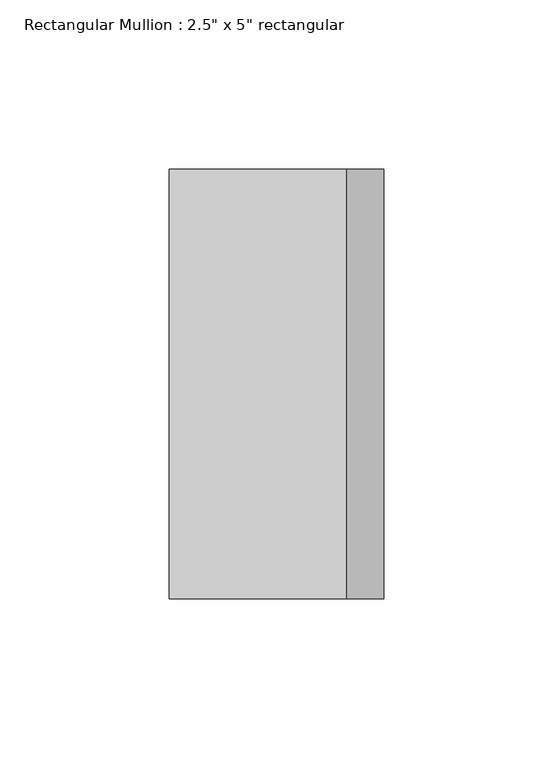
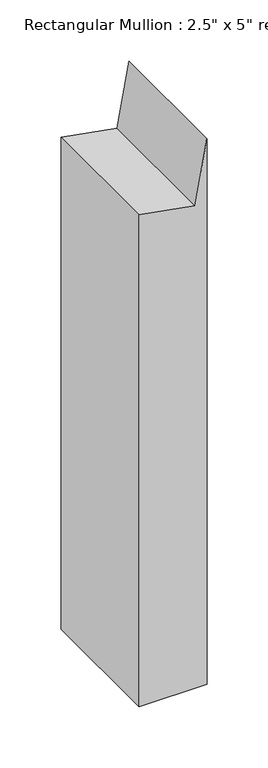
"""IFC4 building model written with IfcOpenShell, lengths in millimetres: member geometry."""

import ifcopenshell
import ifcopenshell.guid

model = None  # the IFC model being written
_history = None  # IfcOwnerHistory: only IFC2X3 demands one
_inside = {}  # id of a spatial element -> (the spatial element, [elements in it])
_under = {}  # id of a project, library or spatial element -> (it, [spatial elements below it])
_declared = {}  # id of a project -> (the project, [libraries it declares])
_typed = {}  # id of a type object -> (the type object, [elements of that type])
_made_of = {}  # id of a material, layer set ... -> (it, [elements and type objects made of it])


def new_model(schema):
    """Start an empty IFC model of exactly this schema.

    Asked for "IFC4X3", IfcOpenShell would pick the latest addendum, in which some entities
    have other attributes; the version numbers below select the first issue.
    IFC2X3 requires an IfcOwnerHistory on every rooted entity: one is made here for all.
    """
    global model, _history
    if schema == "IFC4X3":
        model = ifcopenshell.file(schema_version=(4, 3, 0, 0))
    else:
        model = ifcopenshell.file(schema=schema)
    _inside.clear()
    _under.clear()
    _declared.clear()
    _typed.clear()
    _made_of.clear()
    _history = None
    if model.schema == "IFC2X3":
        org = make("IfcOrganization", Name="unknown")
        user = make(
            "IfcPersonAndOrganization",
            ThePerson=make("IfcPerson", FamilyName="unknown"),
            TheOrganization=org,
        )
        app = make(
            "IfcApplication",
            ApplicationDeveloper=org,
            Version="unknown",
            ApplicationFullName="unknown",
            ApplicationIdentifier="unknown",
        )
        _history = make(
            "IfcOwnerHistory",
            OwningUser=user,
            OwningApplication=app,
            ChangeAction="ADDED",
            CreationDate=0,
        )
    return model


def make(cls, **values):
    """One entity of the class cls with the attributes given. An attribute that is None is left unset."""
    return model.create_entity(
        cls, **{name: value for name, value in values.items() if value is not None}
    )


def rooted(cls, **values):
    """An entity with a GlobalId (a new one), such as an element, a storey or a relation."""
    return make(cls, GlobalId=ifcopenshell.guid.new(), OwnerHistory=_history, **values)


def si_unit(unit_type, name, prefix=None):
    """IfcSIUnit, for example si_unit("LENGTHUNIT", "METRE", prefix="MILLI")."""
    return make("IfcSIUnit", UnitType=unit_type, Prefix=prefix, Name=name)


def assignment(units):
    """IfcUnitAssignment: the units of a project."""
    return None if units is None else make("IfcUnitAssignment", Units=units)


def point(xyz):
    """IfcCartesianPoint."""
    return None if xyz is None else make("IfcCartesianPoint", Coordinates=xyz)


def direction(xyz):
    """IfcDirection."""
    return None if xyz is None else make("IfcDirection", DirectionRatios=xyz)


def frame(location, z_axis=None, x_axis=None):
    """IfcAxis2Placement3D, a coordinate frame: its origin and axes. An axis left out is left unset."""
    return make(
        "IfcAxis2Placement3D",
        Location=point(location),
        Axis=direction(z_axis),
        RefDirection=direction(x_axis),
    )


def origin():
    """The frame at (0, 0, 0) with its axes left unset."""
    return frame((0.0, 0.0, 0.0))


def place(relative_to, where):
    """IfcLocalPlacement: puts the frame where relative to a parent placement (None: the world)."""
    return make(
        "IfcLocalPlacement", PlacementRelTo=relative_to, RelativePlacement=where
    )


def context(
    kind, dimensions, precision=None, world=None, true_north=None, identifier=None
):
    """IfcGeometricRepresentationContext, for example the 3D "Model" context."""
    return make(
        "IfcGeometricRepresentationContext",
        ContextIdentifier=identifier,
        ContextType=kind,
        CoordinateSpaceDimension=dimensions,
        Precision=precision,
        WorldCoordinateSystem=world,
        TrueNorth=true_north,
    )


def project(units=None, contexts=None):
    """IfcProject with its units and contexts."""
    return rooted(
        "IfcProject",
        Name="project",
        RepresentationContexts=contexts,
        UnitsInContext=assignment(units),
    )


def spatial(cls, under=None, at=None, **own):
    """A site, building, storey or space (cls), placed at a placement, below another one or the project."""
    s = rooted(cls, ObjectPlacement=at, **own)
    if under is not None:
        _under.setdefault(under.id(), (under, []))[1].append(s)
    return s


def polyline(points):
    """IfcPolyline through the points."""
    return make("IfcPolyline", Points=[point(p) for p in points])


def outline(outer, holes=None, kind="AREA"):
    """IfcArbitraryClosedProfileDef: a profile drawn as a closed curve; with holes, ...WithVoids."""
    if holes is None:
        return make("IfcArbitraryClosedProfileDef", ProfileType=kind, OuterCurve=outer)
    return make(
        "IfcArbitraryProfileDefWithVoids",
        ProfileType=kind,
        OuterCurve=outer,
        InnerCurves=holes,
    )


def extrude(swept, where, along, depth):
    """IfcExtrudedAreaSolid: the profile swept, set in the frame where, extruded along a direction by depth."""
    return make(
        "IfcExtrudedAreaSolid",
        SweptArea=swept,
        Position=where,
        ExtrudedDirection=direction(along),
        Depth=depth,
    )


def shape(context_of_items, identifier, shape_type, items):
    """IfcShapeRepresentation: the items that make up one representation, for example the "Body"."""
    return make(
        "IfcShapeRepresentation",
        ContextOfItems=context_of_items,
        RepresentationIdentifier=identifier,
        RepresentationType=shape_type,
        Items=items,
    )


def source(mapping_origin, context_of_items, identifier, shape_type, items):
    """IfcRepresentationMap: a shape defined once, which mapped items show again and again."""
    return make(
        "IfcRepresentationMap",
        MappingOrigin=mapping_origin,
        MappedRepresentation=shape(context_of_items, identifier, shape_type, items),
    )


def transform(
    local_origin,
    x_axis=None,
    y_axis=None,
    z_axis=None,
    scale=None,
    scale2=None,
    scale3=None,
    uniform=True,
):
    """IfcCartesianTransformationOperator3D, or its non-uniform kind. x_axis, y_axis, z_axis: its Axis1, 2, 3."""
    if uniform:
        return make(
            "IfcCartesianTransformationOperator3D",
            Axis1=direction(x_axis),
            Axis2=direction(y_axis),
            LocalOrigin=point(local_origin),
            Scale=scale,
            Axis3=direction(z_axis),
        )
    return make(
        "IfcCartesianTransformationOperator3DnonUniform",
        Axis1=direction(x_axis),
        Axis2=direction(y_axis),
        LocalOrigin=point(local_origin),
        Scale=scale,
        Axis3=direction(z_axis),
        Scale2=scale2,
        Scale3=scale3,
    )


def mapped(mapping_source, mapping_target):
    """IfcMappedItem: shows the shape of a source again, moved by a transform."""
    return make(
        "IfcMappedItem", MappingSource=mapping_source, MappingTarget=mapping_target
    )


def made_of(thing, what):
    """Note that an element or type object is made of a material, layer set ...; save() writes the relation."""
    if what is not None:
        _made_of.setdefault(what.id(), (what, []))[1].append(thing)
    return thing


def element(
    cls,
    number,
    at=None,
    inside=None,
    cuts=None,
    type_object=None,
    material=None,
    context=None,
    identifier="Body",
    shape_type=None,
    held_by="IfcProductDefinitionShape",
    body=None,
    shapes=None,
    **own,
):
    """One element of the class cls, such as IfcWall. Its Tag is "e" and its number.

    at: its placement. inside: the storey or other place that contains it. cuts: it is an
    opening in that element (IfcRelVoidsElement). A single representation is given by context,
    identifier, shape_type and body (its items); several are given by shapes. held_by: the class
    of the entity that holds the representations. save() writes the other relations.
    """
    e = rooted(cls, Tag="e%d" % number, ObjectPlacement=at, **own)
    if body is not None:
        shapes = [shape(context, identifier, shape_type, body)]
    if shapes is not None:
        e.Representation = make(held_by, Representations=shapes)
    if inside is not None:
        _inside.setdefault(inside.id(), (inside, []))[1].append(e)
    if cuts is not None:
        rooted(
            "IfcRelVoidsElement", RelatingBuildingElement=cuts, RelatedOpeningElement=e
        )
    if type_object is not None:
        _typed.setdefault(type_object.id(), (type_object, []))[1].append(e)
    return made_of(e, material)


def aggregate(whole, parts):
    """IfcRelAggregates: a whole, such as a stair, and the parts it consists of."""
    return rooted("IfcRelAggregates", RelatingObject=whole, RelatedObjects=parts)


def save(model, path):
    """Write the relations noted so far, then the file.

    IfcRelAggregates (storeys below a building ...), IfcRelContainedInSpatialStructure (elements
    in a storey), IfcRelDefinesByType, IfcRelAssociatesMaterial and IfcRelDeclares: one each for
    every whole, place, type object, material and project.
    """
    for whole, parts in _under.values():
        aggregate(whole, parts)
    for where, things in _inside.values():
        rooted(
            "IfcRelContainedInSpatialStructure",
            RelatedElements=things,
            RelatingStructure=where,
        )
    for kind, things in _typed.values():
        rooted("IfcRelDefinesByType", RelatedObjects=things, RelatingType=kind)
    for what, things in _made_of.values():
        rooted("IfcRelAssociatesMaterial", RelatedObjects=things, RelatingMaterial=what)
    for by, libraries in _declared.values():
        rooted("IfcRelDeclares", RelatingContext=by, RelatedDefinitions=libraries)
    model.write(path)


def member_2b5633e6(model_context):
    return source(origin(), model_context, "Body", "SweptSolid", [
        extrude(outline(polyline([(0.0, 0.0), (-62.5352923, -11.0266593), (-53.2828266, -63.5), (-541.6285548, -63.5), (-541.6285548, 0.0), (0.0, 0.0)])), frame((0.0, -63.5, 0.0), z_axis=(0.0, 1.0, 0.0), x_axis=(0.0, 0.0, 1.0)), (0.0, 0.0, 1.0), 127.0),
    ])


if __name__ == "__main__":
    model = new_model("IFC4")
    model_context = context("Model", 3, world=origin())
    ifc_project = project(units=[si_unit("LENGTHUNIT", "METRE", prefix="MILLI")], contexts=[model_context])
    site = spatial("IfcSite", under=ifc_project)
    building = spatial("IfcBuilding", under=site)
    placement = place(None, origin())
    member_shape = member_2b5633e6(model_context)
    element("IfcMember", 1, ObjectType="Rectangular Mullion : 2.5\" x 5\" rectangular", at=placement, inside=building, context=model_context, shape_type="MappedRepresentation", body=[
        mapped(member_shape, transform((0.0, 0.0, 0.0), x_axis=(1.0, 0.0, 0.0), y_axis=(0.0, 1.0, 0.0), z_axis=(0.0, 0.0, 1.0))),
    ])
    save(model, "model.ifc")

# Revit data of these elements
# Project information
#   SR Document GUID = "d36f5d78-752a-40d6-a009-b379f065f3eb"
# Type "Rectangular Mullion : 2.5\" x 5\" rectangular"
#   built-in parameter 1007304 = 0.416667 (stored number, unit not read)
#   built-in parameter 1007301 = 0.104167 (stored number, unit not read)
#   built-in parameter 1007300 = 0.104167 (stored number, unit not read)
# Element 1 (IfcMember, "Rectangular Mullion : 2.5\" x 5\" rectangular")
#   Materials on its faces: "Black Mullions"
# Materials
#   "Black Mullions": class "Wood", colour RGB 0 0 0, transparency 0, Cost = 0
